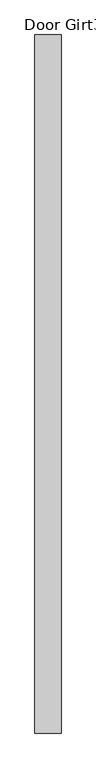
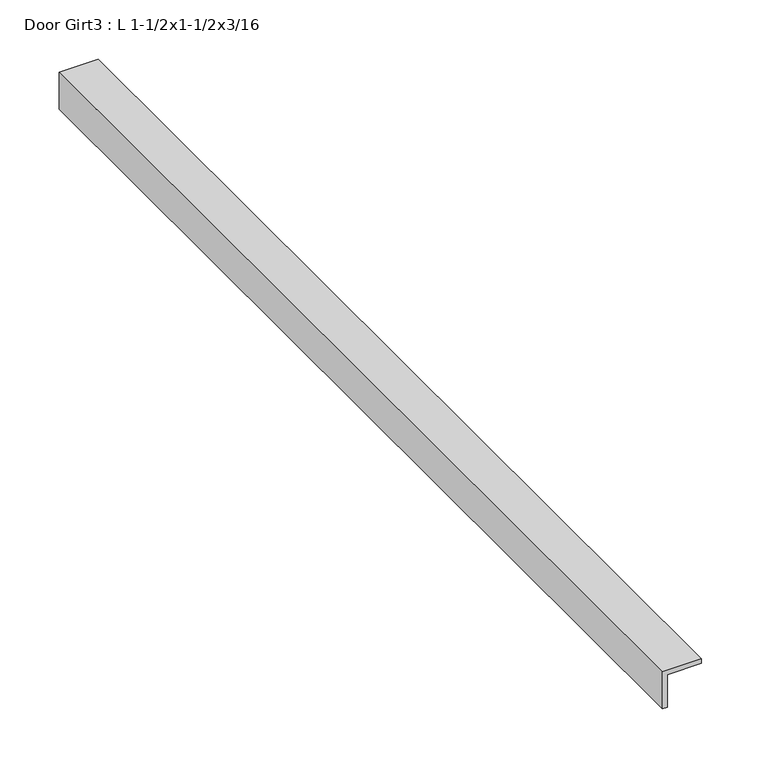
"""IFC4 building model written with IfcOpenShell, lengths in millimetres: proxy geometry, Door Girt3 : L 1-1/2x1-1/2x3/16."""

from ifc_helpers import new_model, si_unit, frame, origin, place, context, project, spatial, polyline, outline, extrude, source, transform, mapped, element, save


def door_girt3_l_1_1_2x1_1_2x3_16_9aa2a562(model_context):
    return source(origin(), model_context, "Body", "SweptSolid", [
        extrude(outline(polyline([(812.8, 587403.9934739), (812.8, 587365.8934739), (774.7, 587365.8934739), (774.7, 587370.6559739), (808.0375, 587370.6559739), (808.0375, 587403.9934739), (812.8, 587403.9934739)])), frame((0.0, -536263.6038841, 0.0), z_axis=(0.0, 1.0, 0.0), x_axis=(0.0, 0.0, 1.0)), (0.0, 0.0, 1.0), 1017.5875),
    ])


if __name__ == "__main__":
    model = new_model("IFC4")
    model_context = context("Model", 3, world=origin())
    ifc_project = project(units=[si_unit("LENGTHUNIT", "METRE", prefix="MILLI")], contexts=[model_context])
    site = spatial("IfcSite", under=ifc_project)
    building = spatial("IfcBuilding", under=site)
    placement = place(None, origin())
    door_girt3_l_1_1_2x1_1_2x3_16_shape = door_girt3_l_1_1_2x1_1_2x3_16_9aa2a562(model_context)
    element("IfcBuildingElementProxy", 1, Name="Door Girt3 : L 1-1/2x1-1/2x3/16", ObjectType="Door Girt3 : L 1-1/2x1-1/2x3/16", at=placement, inside=building, context=model_context, shape_type="MappedRepresentation", body=[
        mapped(door_girt3_l_1_1_2x1_1_2x3_16_shape, transform((0.0, 0.0, 0.0), x_axis=(1.0, 0.0, 0.0), y_axis=(0.0, 1.0, 0.0), z_axis=(0.0, 0.0, 1.0))),
    ])
    save(model, "model.ifc")

# Revit data of these elements
# Element 1 (IfcBuildingElementProxy, "Door Girt3 : L 1-1/2x1-1/2x3/16")
#   Materials on its faces: "1-1/2\"X1-1/2\" GALV. STL L"
# Materials
#   "1-1/2\"X1-1/2\" GALV. STL L": class "Generic", colour RGB 211 211 207, transparency 0, Cost = 0
